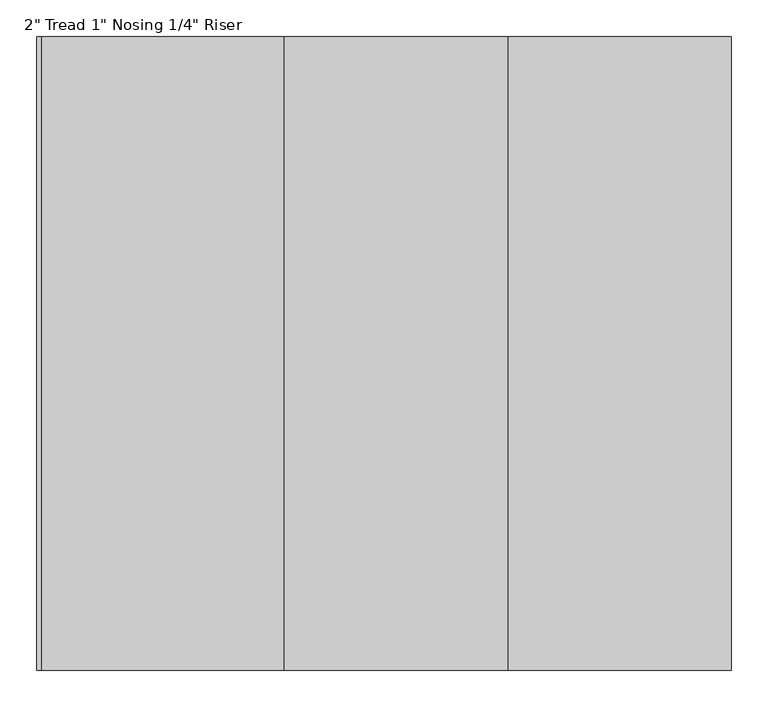
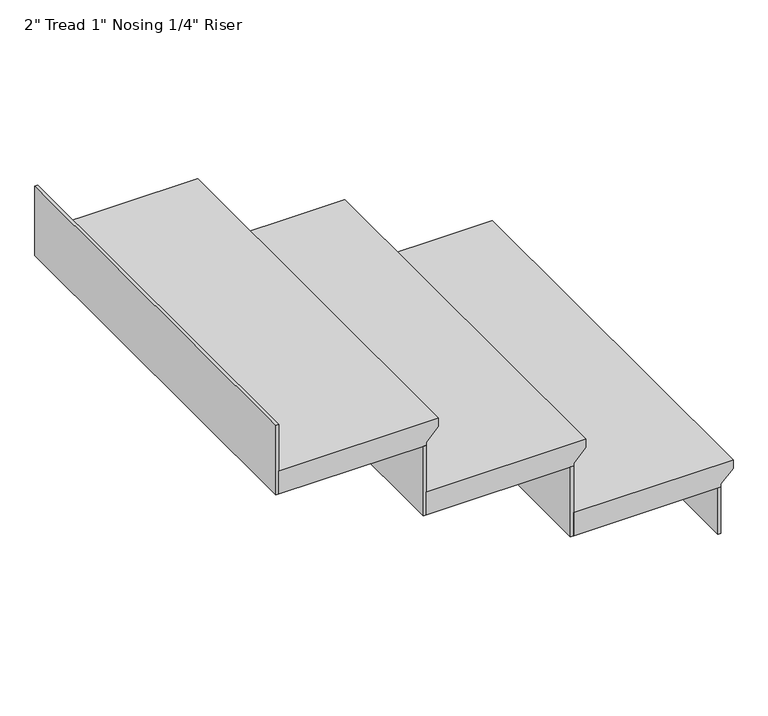
"""IFC4 building model written with IfcOpenShell, lengths in millimetres: stair flight geometry."""

from ifc_helpers import new_model, si_unit, frame, origin, place, context, project, spatial, polyline, outline, extrude, source, transform, mapped, element, save


def stair_flight_42b57d67(model_context):
    return source(origin(), model_context, "Body", "SweptSolid", [
        extrude(outline(polyline([(-406.4, 14036.5848867), (-406.4, 13706.3848867), (-457.2, 13706.3848867), (-457.2, 14011.1848867), (-450.85, 14011.1848867), (-425.45, 14036.5848867), (-406.4, 14036.5848867)])), frame((0.0, 6120.60625, 0.0), z_axis=(0.0, 1.0, 0.0), x_axis=(0.0, 0.0, 1.0)), (0.0, 0.0, 1.0), 863.6),
        extrude(outline(polyline([(14004.8348867, 6984.20625), (14011.1848867, 6984.20625), (14011.1848867, 6120.60625), (14004.8348867, 6120.60625), (14004.8348867, 6984.20625)])), frame((0.0, 0.0, -558.8), z_axis=(0.0, 0.0, 1.0), x_axis=(1.0, 0.0, 0.0)), (0.0, 0.0, 1.0), 101.6),
        extrude(outline(polyline([(13700.0348867, 6984.20625), (13706.3848867, 6984.20625), (13706.3848867, 6120.60625), (13700.0348867, 6120.60625), (13700.0348867, 6984.20625)])), frame((0.0, 0.0, -457.2), z_axis=(0.0, 0.0, 1.0), x_axis=(1.0, 0.0, 0.0)), (0.0, 0.0, 1.0), 152.4),
        extrude(outline(polyline([(-254.0, 13731.7848867), (-254.0, 13401.5848867), (-304.8, 13401.5848867), (-304.8, 13706.3848867), (-298.45, 13706.3848867), (-273.05, 13731.7848867), (-254.0, 13731.7848867)])), frame((0.0, 6120.60625, 0.0), z_axis=(0.0, 1.0, 0.0), x_axis=(0.0, 0.0, 1.0)), (0.0, 0.0, 1.0), 863.6),
        extrude(outline(polyline([(13395.2348867, 6984.20625), (13401.5848867, 6984.20625), (13401.5848867, 6120.60625), (13395.2348867, 6120.60625), (13395.2348867, 6984.20625)])), frame((0.0, 0.0, -304.8), z_axis=(0.0, 0.0, 1.0), x_axis=(1.0, 0.0, 0.0)), (0.0, 0.0, 1.0), 152.4),
        extrude(outline(polyline([(-101.6, 13426.9848867), (-101.6, 13096.7848867), (-152.4, 13096.7848867), (-152.4, 13401.5848867), (-146.05, 13401.5848867), (-120.65, 13426.9848867), (-101.6, 13426.9848867)])), frame((0.0, 6120.60625, 0.0), z_axis=(0.0, 1.0, 0.0), x_axis=(0.0, 0.0, 1.0)), (0.0, 0.0, 1.0), 863.6),
        extrude(outline(polyline([(13090.4348867, 6984.20625), (13096.7848867, 6984.20625), (13096.7848867, 6120.60625), (13090.4348867, 6120.60625), (13090.4348867, 6984.20625)])), frame((0.0, 0.0, -152.4), z_axis=(0.0, 0.0, 1.0), x_axis=(1.0, 0.0, 0.0)), (0.0, 0.0, 1.0), 152.4),
    ])


if __name__ == "__main__":
    model = new_model("IFC4")
    model_context = context("Model", 3, world=origin())
    ifc_project = project(units=[si_unit("LENGTHUNIT", "METRE", prefix="MILLI")], contexts=[model_context])
    site = spatial("IfcSite", under=ifc_project)
    building = spatial("IfcBuilding", under=site)
    placement = place(None, origin())
    stair_flight_shape = stair_flight_42b57d67(model_context)
    element("IfcStairFlight", 1, ObjectType="2\" Tread 1\" Nosing 1/4\" Riser", at=placement, inside=building, context=model_context, shape_type="MappedRepresentation", body=[
        mapped(stair_flight_shape, transform((0.0, 0.0, 0.0), x_axis=(1.0, 0.0, 0.0), y_axis=(0.0, 1.0, 0.0), z_axis=(0.0, 0.0, 1.0))),
    ])
    save(model, "model.ifc")
